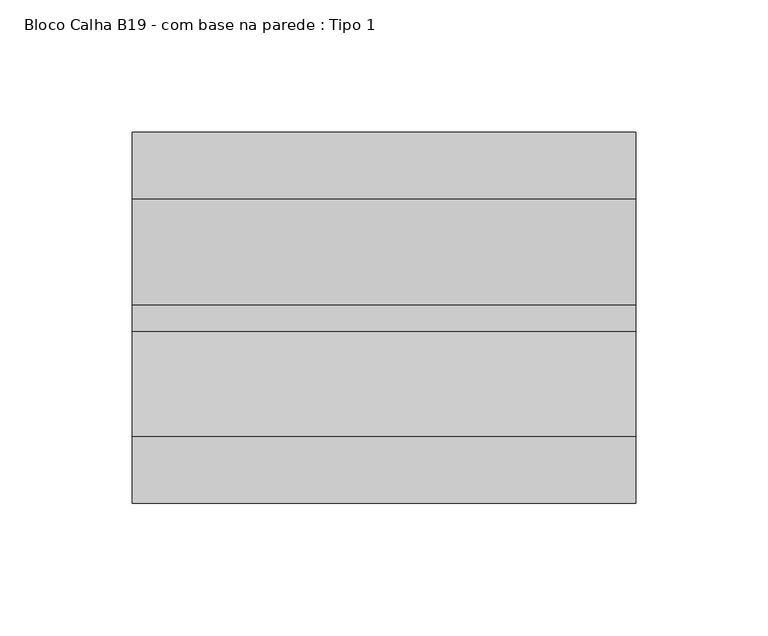
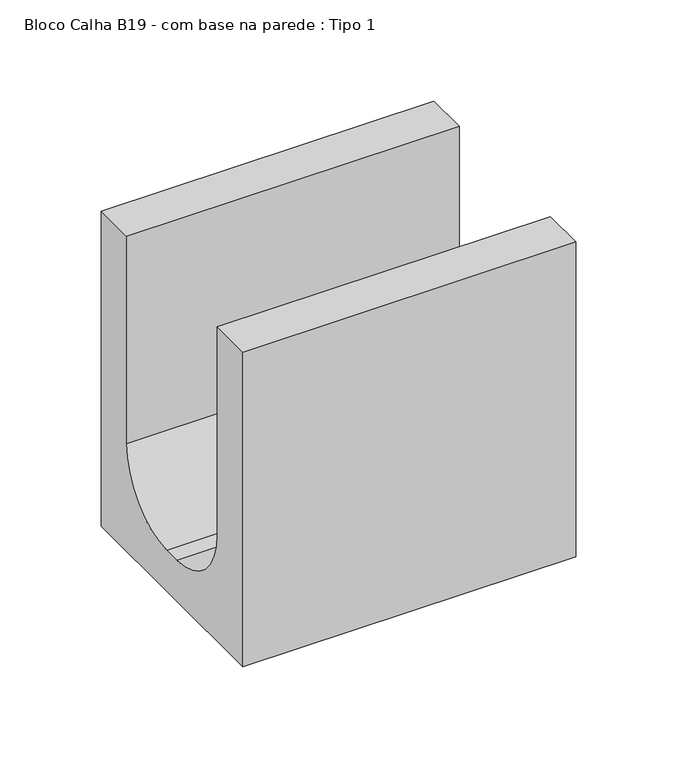
"""IFC4 building model written with IfcOpenShell, lengths in millimetres: proxy geometry, Bloco Calha B19 - com base na parede : Tipo 1."""

from ifc_helpers import new_model, si_unit, point, frame, frame_2d, origin, place, context, project, spatial, polyline, circle_curve, trimmed, segment, composite_curve, outline, extrude, source, transform, mapped, element, save


def bloco_calha_b19_com_base_na_parede_tipo_1_0c22f821(model_context):
    return source(origin(), model_context, "Body", "SweptSolid", [
        extrude(outline(composite_curve([segment(polyline([(-70.0, 0.0), (-70.0, 190.0), (-45.0, 190.0), (-45.0, 65.0)]), True, "CONTINUOUS"), segment(trimmed(circle_curve(frame_2d((-5.0, 65.0)), 40.0), [point((-45.0, 65.0))], [point((-5.0, 25.0))], True, "CARTESIAN"), True, "CONTINUOUS"), segment(polyline([(-5.0, 25.0), (5.0, 25.0)]), True, "CONTINUOUS"), segment(trimmed(circle_curve(frame_2d((5.0, 65.0)), 40.0), [point((5.0, 25.0))], [point((45.0, 65.0))], True, "CARTESIAN"), True, "CONTINUOUS"), segment(polyline([(45.0, 65.0), (45.0, 190.0), (70.0, 190.0), (70.0, 0.0), (-70.0, 0.0)]), True, "CONTINUOUS")], self_intersect=False)), frame((30.0, 0.0, 0.0), z_axis=(1.0, 0.0, 0.0), x_axis=(0.0, 1.0, 0.0)), (0.0, 0.0, 1.0), 190.0),
    ])


if __name__ == "__main__":
    model = new_model("IFC4")
    model_context = context("Model", 3, world=origin())
    ifc_project = project(units=[si_unit("LENGTHUNIT", "METRE", prefix="MILLI")], contexts=[model_context])
    site = spatial("IfcSite", under=ifc_project)
    building = spatial("IfcBuilding", under=site)
    placement = place(None, origin())
    bloco_calha_b19_com_base_na_parede_tipo_1_shape = bloco_calha_b19_com_base_na_parede_tipo_1_0c22f821(model_context)
    element("IfcBuildingElementProxy", 1, Name="Bloco Calha B19 - com base na parede : Tipo 1", ObjectType="Bloco Calha B19 - com base na parede : Tipo 1", at=placement, inside=building, context=model_context, shape_type="MappedRepresentation", body=[
        mapped(bloco_calha_b19_com_base_na_parede_tipo_1_shape, transform((0.0, 0.0, 0.0), x_axis=(1.0, 0.0, 0.0), y_axis=(0.0, 1.0, 0.0), z_axis=(0.0, 0.0, 1.0))),
    ])
    save(model, "model.ifc")

# Revit data of these elements
# Type "Bloco Calha B19 - com base na parede : Tipo 1"
#   SINAPI = ""
#   Assembly Code = ""
